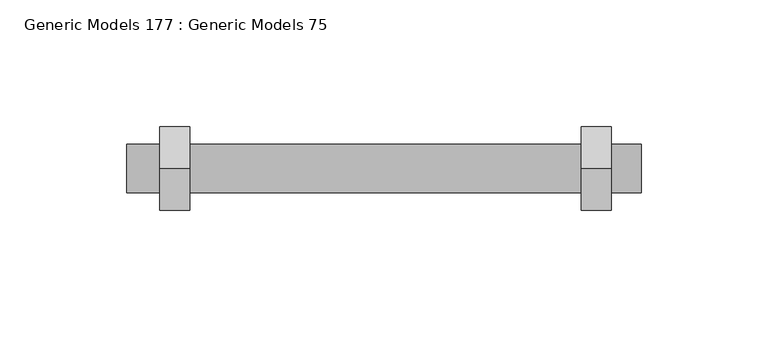
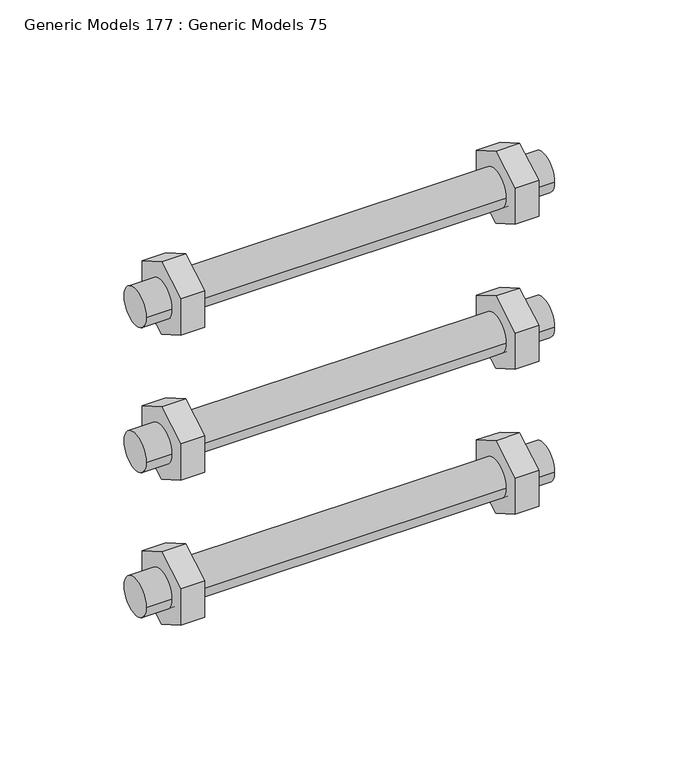
"""IFC4 building model written with IfcOpenShell, lengths in millimetres: proxy geometry, Generic Models 177 : Generic Models 75."""

import ifcopenshell
import ifcopenshell.guid

model = None  # the IFC model being written
_history = None  # IfcOwnerHistory: only IFC2X3 demands one
_inside = {}  # id of a spatial element -> (the spatial element, [elements in it])
_under = {}  # id of a project, library or spatial element -> (it, [spatial elements below it])
_declared = {}  # id of a project -> (the project, [libraries it declares])
_typed = {}  # id of a type object -> (the type object, [elements of that type])
_made_of = {}  # id of a material, layer set ... -> (it, [elements and type objects made of it])


def new_model(schema):
    """Start an empty IFC model of exactly this schema.

    Asked for "IFC4X3", IfcOpenShell would pick the latest addendum, in which some entities
    have other attributes; the version numbers below select the first issue.
    IFC2X3 requires an IfcOwnerHistory on every rooted entity: one is made here for all.
    """
    global model, _history
    if schema == "IFC4X3":
        model = ifcopenshell.file(schema_version=(4, 3, 0, 0))
    else:
        model = ifcopenshell.file(schema=schema)
    _inside.clear()
    _under.clear()
    _declared.clear()
    _typed.clear()
    _made_of.clear()
    _history = None
    if model.schema == "IFC2X3":
        org = make("IfcOrganization", Name="unknown")
        user = make(
            "IfcPersonAndOrganization",
            ThePerson=make("IfcPerson", FamilyName="unknown"),
            TheOrganization=org,
        )
        app = make(
            "IfcApplication",
            ApplicationDeveloper=org,
            Version="unknown",
            ApplicationFullName="unknown",
            ApplicationIdentifier="unknown",
        )
        _history = make(
            "IfcOwnerHistory",
            OwningUser=user,
            OwningApplication=app,
            ChangeAction="ADDED",
            CreationDate=0,
        )
    return model


def make(cls, **values):
    """One entity of the class cls with the attributes given. An attribute that is None is left unset."""
    return model.create_entity(
        cls, **{name: value for name, value in values.items() if value is not None}
    )


def rooted(cls, **values):
    """An entity with a GlobalId (a new one), such as an element, a storey or a relation."""
    return make(cls, GlobalId=ifcopenshell.guid.new(), OwnerHistory=_history, **values)


def si_unit(unit_type, name, prefix=None):
    """IfcSIUnit, for example si_unit("LENGTHUNIT", "METRE", prefix="MILLI")."""
    return make("IfcSIUnit", UnitType=unit_type, Prefix=prefix, Name=name)


def assignment(units):
    """IfcUnitAssignment: the units of a project."""
    return None if units is None else make("IfcUnitAssignment", Units=units)


def point(xyz):
    """IfcCartesianPoint."""
    return None if xyz is None else make("IfcCartesianPoint", Coordinates=xyz)


def direction(xyz):
    """IfcDirection."""
    return None if xyz is None else make("IfcDirection", DirectionRatios=xyz)


def frame(location, z_axis=None, x_axis=None):
    """IfcAxis2Placement3D, a coordinate frame: its origin and axes. An axis left out is left unset."""
    return make(
        "IfcAxis2Placement3D",
        Location=point(location),
        Axis=direction(z_axis),
        RefDirection=direction(x_axis),
    )


def frame_2d(location, x_axis=None):
    """IfcAxis2Placement2D, a coordinate frame in the plane: its origin and x axis."""
    return make(
        "IfcAxis2Placement2D", Location=point(location), RefDirection=direction(x_axis)
    )


def origin():
    """The frame at (0, 0, 0) with its axes left unset."""
    return frame((0.0, 0.0, 0.0))


def place(relative_to, where):
    """IfcLocalPlacement: puts the frame where relative to a parent placement (None: the world)."""
    return make(
        "IfcLocalPlacement", PlacementRelTo=relative_to, RelativePlacement=where
    )


def context(
    kind, dimensions, precision=None, world=None, true_north=None, identifier=None
):
    """IfcGeometricRepresentationContext, for example the 3D "Model" context."""
    return make(
        "IfcGeometricRepresentationContext",
        ContextIdentifier=identifier,
        ContextType=kind,
        CoordinateSpaceDimension=dimensions,
        Precision=precision,
        WorldCoordinateSystem=world,
        TrueNorth=true_north,
    )


def project(units=None, contexts=None):
    """IfcProject with its units and contexts."""
    return rooted(
        "IfcProject",
        Name="project",
        RepresentationContexts=contexts,
        UnitsInContext=assignment(units),
    )


def spatial(cls, under=None, at=None, **own):
    """A site, building, storey or space (cls), placed at a placement, below another one or the project."""
    s = rooted(cls, ObjectPlacement=at, **own)
    if under is not None:
        _under.setdefault(under.id(), (under, []))[1].append(s)
    return s


def polyline(points):
    """IfcPolyline through the points."""
    return make("IfcPolyline", Points=[point(p) for p in points])


def circle_curve(where, radius):
    """IfcCircle in the frame where."""
    return make("IfcCircle", Position=where, Radius=radius)


def trimmed(basis, trim1, trim2, sense, master):
    """IfcTrimmedCurve: the piece of a basis curve between two trims."""
    return make(
        "IfcTrimmedCurve",
        BasisCurve=basis,
        Trim1=trim1,
        Trim2=trim2,
        SenseAgreement=sense,
        MasterRepresentation=master,
    )


def segment(curve, same_sense, transition):
    """IfcCompositeCurveSegment."""
    return make(
        "IfcCompositeCurveSegment",
        Transition=transition,
        SameSense=same_sense,
        ParentCurve=curve,
    )


def composite_curve(segments, self_intersect=None):
    """IfcCompositeCurve: segments joined end to end."""
    return make("IfcCompositeCurve", Segments=segments, SelfIntersect=self_intersect)


def outline(outer, holes=None, kind="AREA"):
    """IfcArbitraryClosedProfileDef: a profile drawn as a closed curve; with holes, ...WithVoids."""
    if holes is None:
        return make("IfcArbitraryClosedProfileDef", ProfileType=kind, OuterCurve=outer)
    return make(
        "IfcArbitraryProfileDefWithVoids",
        ProfileType=kind,
        OuterCurve=outer,
        InnerCurves=holes,
    )


def extrude(swept, where, along, depth):
    """IfcExtrudedAreaSolid: the profile swept, set in the frame where, extruded along a direction by depth."""
    return make(
        "IfcExtrudedAreaSolid",
        SweptArea=swept,
        Position=where,
        ExtrudedDirection=direction(along),
        Depth=depth,
    )


def shape(context_of_items, identifier, shape_type, items):
    """IfcShapeRepresentation: the items that make up one representation, for example the "Body"."""
    return make(
        "IfcShapeRepresentation",
        ContextOfItems=context_of_items,
        RepresentationIdentifier=identifier,
        RepresentationType=shape_type,
        Items=items,
    )


def source(mapping_origin, context_of_items, identifier, shape_type, items):
    """IfcRepresentationMap: a shape defined once, which mapped items show again and again."""
    return make(
        "IfcRepresentationMap",
        MappingOrigin=mapping_origin,
        MappedRepresentation=shape(context_of_items, identifier, shape_type, items),
    )


def transform(
    local_origin,
    x_axis=None,
    y_axis=None,
    z_axis=None,
    scale=None,
    scale2=None,
    scale3=None,
    uniform=True,
):
    """IfcCartesianTransformationOperator3D, or its non-uniform kind. x_axis, y_axis, z_axis: its Axis1, 2, 3."""
    if uniform:
        return make(
            "IfcCartesianTransformationOperator3D",
            Axis1=direction(x_axis),
            Axis2=direction(y_axis),
            LocalOrigin=point(local_origin),
            Scale=scale,
            Axis3=direction(z_axis),
        )
    return make(
        "IfcCartesianTransformationOperator3DnonUniform",
        Axis1=direction(x_axis),
        Axis2=direction(y_axis),
        LocalOrigin=point(local_origin),
        Scale=scale,
        Axis3=direction(z_axis),
        Scale2=scale2,
        Scale3=scale3,
    )


def mapped(mapping_source, mapping_target):
    """IfcMappedItem: shows the shape of a source again, moved by a transform."""
    return make(
        "IfcMappedItem", MappingSource=mapping_source, MappingTarget=mapping_target
    )


def made_of(thing, what):
    """Note that an element or type object is made of a material, layer set ...; save() writes the relation."""
    if what is not None:
        _made_of.setdefault(what.id(), (what, []))[1].append(thing)
    return thing


def element(
    cls,
    number,
    at=None,
    inside=None,
    cuts=None,
    type_object=None,
    material=None,
    context=None,
    identifier="Body",
    shape_type=None,
    held_by="IfcProductDefinitionShape",
    body=None,
    shapes=None,
    **own,
):
    """One element of the class cls, such as IfcWall. Its Tag is "e" and its number.

    at: its placement. inside: the storey or other place that contains it. cuts: it is an
    opening in that element (IfcRelVoidsElement). A single representation is given by context,
    identifier, shape_type and body (its items); several are given by shapes. held_by: the class
    of the entity that holds the representations. save() writes the other relations.
    """
    e = rooted(cls, Tag="e%d" % number, ObjectPlacement=at, **own)
    if body is not None:
        shapes = [shape(context, identifier, shape_type, body)]
    if shapes is not None:
        e.Representation = make(held_by, Representations=shapes)
    if inside is not None:
        _inside.setdefault(inside.id(), (inside, []))[1].append(e)
    if cuts is not None:
        rooted(
            "IfcRelVoidsElement", RelatingBuildingElement=cuts, RelatedOpeningElement=e
        )
    if type_object is not None:
        _typed.setdefault(type_object.id(), (type_object, []))[1].append(e)
    return made_of(e, material)


def aggregate(whole, parts):
    """IfcRelAggregates: a whole, such as a stair, and the parts it consists of."""
    return rooted("IfcRelAggregates", RelatingObject=whole, RelatedObjects=parts)


def save(model, path):
    """Write the relations noted so far, then the file.

    IfcRelAggregates (storeys below a building ...), IfcRelContainedInSpatialStructure (elements
    in a storey), IfcRelDefinesByType, IfcRelAssociatesMaterial and IfcRelDeclares: one each for
    every whole, place, type object, material and project.
    """
    for whole, parts in _under.values():
        aggregate(whole, parts)
    for where, things in _inside.values():
        rooted(
            "IfcRelContainedInSpatialStructure",
            RelatedElements=things,
            RelatingStructure=where,
        )
    for kind, things in _typed.values():
        rooted("IfcRelDefinesByType", RelatedObjects=things, RelatingType=kind)
    for what, things in _made_of.values():
        rooted("IfcRelAssociatesMaterial", RelatedObjects=things, RelatingMaterial=what)
    for by, libraries in _declared.values():
        rooted("IfcRelDeclares", RelatingContext=by, RelatedDefinitions=libraries)
    model.write(path)


def generic_models_177_generic_models_75_64a4723a(model_context):
    return source(origin(), model_context, "Body", "SweptSolid", [
        extrude(outline(polyline([(30651.9321951, 271852.097122), (30651.9321951, 271833.047122), (30635.4344112, 271823.522122), (30618.9366273, 271833.047122), (30618.9366273, 271852.097122), (30635.4344112, 271861.622122), (30651.9321951, 271852.097122)])), frame((31918.2596032, 0.0, 0.0), z_axis=(1.0, 0.0, 0.0), x_axis=(0.0, 1.0, 0.0)), (0.0, 0.0, 1.0), 11.90625),
        extrude(outline(polyline([(30651.9321951, 271775.897122), (30651.9321951, 271756.847122), (30635.4344112, 271747.322122), (30618.9366273, 271756.847122), (30618.9366273, 271775.897122), (30635.4344112, 271785.422122), (30651.9321951, 271775.897122)])), frame((31918.2596032, 0.0, 0.0), z_axis=(1.0, 0.0, 0.0), x_axis=(0.0, 1.0, 0.0)), (0.0, 0.0, 1.0), 11.90625),
        extrude(outline(polyline([(30651.9321951, 271699.697122), (30651.9321951, 271680.647122), (30635.4344112, 271671.122122), (30618.9366273, 271680.647122), (30618.9366273, 271699.697122), (30635.4344112, 271709.222122), (30651.9321951, 271699.697122)])), frame((31918.2596032, 0.0, 0.0), z_axis=(1.0, 0.0, 0.0), x_axis=(0.0, 1.0, 0.0)), (0.0, 0.0, 1.0), 11.90625),
        extrude(outline(polyline([(30651.9321951, 271852.097122), (30651.9321951, 271833.047122), (30635.4344112, 271823.522122), (30618.9366273, 271833.047122), (30618.9366273, 271852.097122), (30635.4344112, 271861.622122), (30651.9321951, 271852.097122)])), frame((31751.9689782, 0.0, 0.0), z_axis=(1.0, 0.0, 0.0), x_axis=(0.0, 1.0, 0.0)), (0.0, 0.0, 1.0), 11.90625),
        extrude(outline(polyline([(30651.9321951, 271775.897122), (30651.9321951, 271756.847122), (30635.4344112, 271747.322122), (30618.9366273, 271756.847122), (30618.9366273, 271775.897122), (30635.4344112, 271785.422122), (30651.9321951, 271775.897122)])), frame((31751.9689782, 0.0, 0.0), z_axis=(1.0, 0.0, 0.0), x_axis=(0.0, 1.0, 0.0)), (0.0, 0.0, 1.0), 11.90625),
        extrude(outline(polyline([(30651.9321951, 271699.697122), (30651.9321951, 271680.647122), (30635.4344112, 271671.122122), (30618.9366273, 271680.647122), (30618.9366273, 271699.697122), (30635.4344112, 271709.222122), (30651.9321951, 271699.697122)])), frame((31751.9689782, 0.0, 0.0), z_axis=(1.0, 0.0, 0.0), x_axis=(0.0, 1.0, 0.0)), (0.0, 0.0, 1.0), 11.90625),
        extrude(outline(composite_curve([segment(trimmed(circle_curve(frame_2d((30635.4344112, 271766.372122)), 9.525), [point((30625.9094112, 271766.372122))], [point((30644.9594112, 271766.372122))], False, "CARTESIAN"), True, "CONTINUOUS"), segment(trimmed(circle_curve(frame_2d((30635.4344112, 271766.372122)), 9.525), [point((30644.9594112, 271766.372122))], [point((30625.9094112, 271766.372122))], False, "CARTESIAN"), True, "CONTINUOUS")], self_intersect=False)), frame((31738.8721032, 0.0, 0.0), z_axis=(1.0, 0.0, 0.0), x_axis=(0.0, 1.0, 0.0)), (0.0, 0.0, 1.0), 203.2),
        extrude(outline(composite_curve([segment(trimmed(circle_curve(frame_2d((30635.4344112, 271690.172122)), 9.525), [point((30625.9094112, 271690.172122))], [point((30644.9594112, 271690.172122))], False, "CARTESIAN"), True, "CONTINUOUS"), segment(trimmed(circle_curve(frame_2d((30635.4344112, 271690.172122)), 9.525), [point((30644.9594112, 271690.172122))], [point((30625.9094112, 271690.172122))], False, "CARTESIAN"), True, "CONTINUOUS")], self_intersect=False)), frame((31738.8721032, 0.0, 0.0), z_axis=(1.0, 0.0, 0.0), x_axis=(0.0, 1.0, 0.0)), (0.0, 0.0, 1.0), 203.2),
        extrude(outline(composite_curve([segment(trimmed(circle_curve(frame_2d((30635.4344112, 271842.572122)), 9.525), [point((30625.9094112, 271842.572122))], [point((30644.9594112, 271842.572122))], False, "CARTESIAN"), True, "CONTINUOUS"), segment(trimmed(circle_curve(frame_2d((30635.4344112, 271842.572122)), 9.525), [point((30644.9594112, 271842.572122))], [point((30625.9094112, 271842.572122))], False, "CARTESIAN"), True, "CONTINUOUS")], self_intersect=False)), frame((31738.8721032, 0.0, 0.0), z_axis=(1.0, 0.0, 0.0), x_axis=(0.0, 1.0, 0.0)), (0.0, 0.0, 1.0), 203.2),
    ])


if __name__ == "__main__":
    model = new_model("IFC4")
    model_context = context("Model", 3, world=origin())
    ifc_project = project(units=[si_unit("LENGTHUNIT", "METRE", prefix="MILLI")], contexts=[model_context])
    site = spatial("IfcSite", under=ifc_project)
    building = spatial("IfcBuilding", under=site)
    placement = place(None, origin())
    generic_models_177_generic_models_75_shape = generic_models_177_generic_models_75_64a4723a(model_context)
    element("IfcBuildingElementProxy", 1, Name="Generic Models 177 : Generic Models 75", ObjectType="Generic Models 177 : Generic Models 75", at=placement, inside=building, context=model_context, shape_type="MappedRepresentation", body=[
        mapped(generic_models_177_generic_models_75_shape, transform((0.0, 0.0, 0.0), x_axis=(1.0, 0.0, 0.0), y_axis=(0.0, 1.0, 0.0), z_axis=(0.0, 0.0, 1.0))),
    ])
    save(model, "model.ifc")
